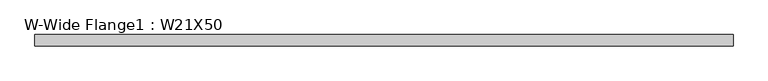
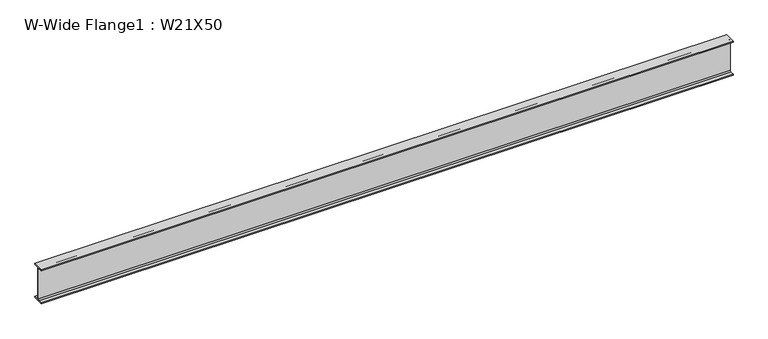
"""IFC4 building model written with IfcOpenShell, lengths in millimetres: beam geometry, W-Wide Flange1 : W21X50."""

from ifc_helpers import new_model, si_unit, point, frame, frame_2d, origin, place, context, project, spatial, polyline, circle_curve, trimmed, segment, composite_curve, outline, extrude, source, transform, mapped, element, save


def w_wide_flange1_w21x50_b251ae41(model_context):
    return source(origin(), model_context, "Body", "SweptSolid", [
        extrude(outline(composite_curve([segment(polyline([(82.931, -250.571), (82.931, -264.16), (-82.931, -264.16), (-82.931, -250.571), (-22.987, -250.571)]), True, "CONTINUOUS"), segment(trimmed(circle_curve(frame_2d((-22.987, -232.41)), 18.161), [point((-22.987, -250.571))], [point((-4.826, -232.41))], True, "CARTESIAN"), True, "CONTINUOUS"), segment(polyline([(-4.826, -232.41), (-4.826, 232.41)]), True, "CONTINUOUS"), segment(trimmed(circle_curve(frame_2d((-22.987, 232.41)), 18.161), [point((-4.826, 232.41))], [point((-22.987, 250.571))], True, "CARTESIAN"), True, "CONTINUOUS"), segment(polyline([(-22.987, 250.571), (-82.931, 250.571), (-82.931, 264.16), (82.931, 264.16), (82.931, 250.571), (22.987, 250.571)]), True, "CONTINUOUS"), segment(trimmed(circle_curve(frame_2d((22.987, 232.41)), 18.161), [point((22.987, 250.571))], [point((4.826, 232.41))], True, "CARTESIAN"), True, "CONTINUOUS"), segment(polyline([(4.826, 232.41), (4.826, -232.41)]), True, "CONTINUOUS"), segment(trimmed(circle_curve(frame_2d((22.987, -232.41)), 18.161), [point((4.826, -232.41))], [point((22.987, -250.571))], True, "CARTESIAN"), True, "CONTINUOUS"), segment(polyline([(22.987, -250.571), (82.931, -250.571)]), True, "CONTINUOUS")], self_intersect=False)), frame((-5047.1365424, 0.0, 0.0), z_axis=(1.0, 0.0, 0.0), x_axis=(0.0, 1.0, 0.0)), (0.0, 0.0, 1.0), 10206.4957372),
    ])


if __name__ == "__main__":
    model = new_model("IFC4")
    model_context = context("Model", 3, world=origin())
    ifc_project = project(units=[si_unit("LENGTHUNIT", "METRE", prefix="MILLI")], contexts=[model_context])
    site = spatial("IfcSite", under=ifc_project)
    building = spatial("IfcBuilding", under=site)
    placement = place(None, origin())
    w_wide_flange1_w21x50_shape = w_wide_flange1_w21x50_b251ae41(model_context)
    element("IfcBeam", 1, ObjectType="W-Wide Flange1 : W21X50", at=placement, inside=building, context=model_context, shape_type="MappedRepresentation", body=[
        mapped(w_wide_flange1_w21x50_shape, transform((0.0, 0.0, 0.0), x_axis=(1.0, 0.0, 0.0), y_axis=(0.0, 1.0, 0.0), z_axis=(0.0, 0.0, 1.0))),
    ])
    save(model, "model.ifc")

# Revit data of these elements
# Type "W-Wide Flange1 : W21X50"
#   Assembly Code = "B10"
#   W = 50
#   Start Extension Calculation [instance default] = 10' - 0"
#   Start Extension [instance default] = -0' - 0 1/2"
#   End Extension Calculation [instance default] = 10' - 0"
#   End Extension [instance default] = -0' - 0 1/2"
#   Length [instance default] = 5' - 0"
#   bf = 0' - 6.53"
#   d = 1' - 8.8"
#   k = 0' - 1 1/4"
#   k2 = 0' - 0.715"
#   tf = 0' - 0.535"
#   tw = 0' - 0.38"
#   A = 0.102083 SF
#   Structural Material [instance default] = Metal - Steel - ASTM A992
# Element 1 (IfcBeam, "W-Wide Flange1 : W21X50")
#   Materials on its faces: "Metal - Steel - ASTM A992"
# Materials
#   "Metal - Steel - ASTM A992": class "Metal", colour RGB 199 199 199, transparency 0
